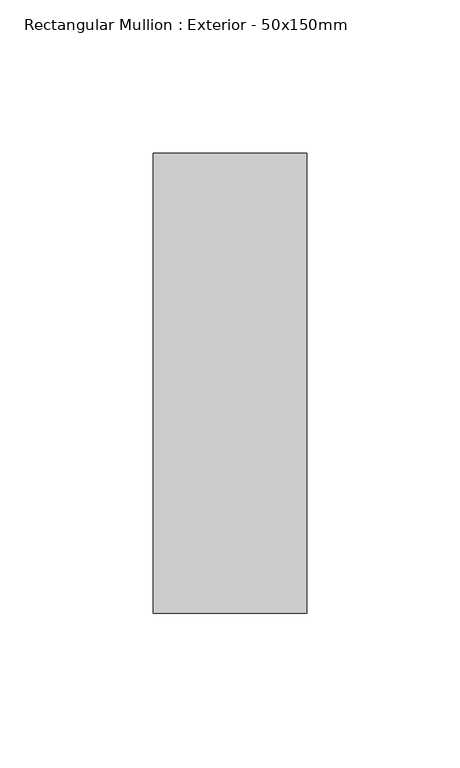
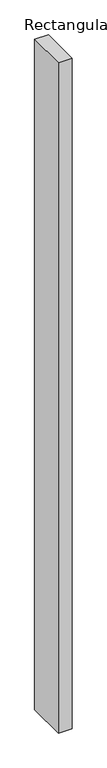
"""IFC4 building model written with IfcOpenShell, lengths in millimetres: member geometry, Rectangular Mullion : Exterior - 50x150mm."""

import ifcopenshell
import ifcopenshell.guid

model = None  # the IFC model being written
_history = None  # IfcOwnerHistory: only IFC2X3 demands one
_inside = {}  # id of a spatial element -> (the spatial element, [elements in it])
_under = {}  # id of a project, library or spatial element -> (it, [spatial elements below it])
_declared = {}  # id of a project -> (the project, [libraries it declares])
_typed = {}  # id of a type object -> (the type object, [elements of that type])
_made_of = {}  # id of a material, layer set ... -> (it, [elements and type objects made of it])


def new_model(schema):
    """Start an empty IFC model of exactly this schema.

    Asked for "IFC4X3", IfcOpenShell would pick the latest addendum, in which some entities
    have other attributes; the version numbers below select the first issue.
    IFC2X3 requires an IfcOwnerHistory on every rooted entity: one is made here for all.
    """
    global model, _history
    if schema == "IFC4X3":
        model = ifcopenshell.file(schema_version=(4, 3, 0, 0))
    else:
        model = ifcopenshell.file(schema=schema)
    _inside.clear()
    _under.clear()
    _declared.clear()
    _typed.clear()
    _made_of.clear()
    _history = None
    if model.schema == "IFC2X3":
        org = make("IfcOrganization", Name="unknown")
        user = make(
            "IfcPersonAndOrganization",
            ThePerson=make("IfcPerson", FamilyName="unknown"),
            TheOrganization=org,
        )
        app = make(
            "IfcApplication",
            ApplicationDeveloper=org,
            Version="unknown",
            ApplicationFullName="unknown",
            ApplicationIdentifier="unknown",
        )
        _history = make(
            "IfcOwnerHistory",
            OwningUser=user,
            OwningApplication=app,
            ChangeAction="ADDED",
            CreationDate=0,
        )
    return model


def make(cls, **values):
    """One entity of the class cls with the attributes given. An attribute that is None is left unset."""
    return model.create_entity(
        cls, **{name: value for name, value in values.items() if value is not None}
    )


def rooted(cls, **values):
    """An entity with a GlobalId (a new one), such as an element, a storey or a relation."""
    return make(cls, GlobalId=ifcopenshell.guid.new(), OwnerHistory=_history, **values)


def si_unit(unit_type, name, prefix=None):
    """IfcSIUnit, for example si_unit("LENGTHUNIT", "METRE", prefix="MILLI")."""
    return make("IfcSIUnit", UnitType=unit_type, Prefix=prefix, Name=name)


def assignment(units):
    """IfcUnitAssignment: the units of a project."""
    return None if units is None else make("IfcUnitAssignment", Units=units)


def point(xyz):
    """IfcCartesianPoint."""
    return None if xyz is None else make("IfcCartesianPoint", Coordinates=xyz)


def direction(xyz):
    """IfcDirection."""
    return None if xyz is None else make("IfcDirection", DirectionRatios=xyz)


def frame(location, z_axis=None, x_axis=None):
    """IfcAxis2Placement3D, a coordinate frame: its origin and axes. An axis left out is left unset."""
    return make(
        "IfcAxis2Placement3D",
        Location=point(location),
        Axis=direction(z_axis),
        RefDirection=direction(x_axis),
    )


def origin():
    """The frame at (0, 0, 0) with its axes left unset."""
    return frame((0.0, 0.0, 0.0))


def place(relative_to, where):
    """IfcLocalPlacement: puts the frame where relative to a parent placement (None: the world)."""
    return make(
        "IfcLocalPlacement", PlacementRelTo=relative_to, RelativePlacement=where
    )


def context(
    kind, dimensions, precision=None, world=None, true_north=None, identifier=None
):
    """IfcGeometricRepresentationContext, for example the 3D "Model" context."""
    return make(
        "IfcGeometricRepresentationContext",
        ContextIdentifier=identifier,
        ContextType=kind,
        CoordinateSpaceDimension=dimensions,
        Precision=precision,
        WorldCoordinateSystem=world,
        TrueNorth=true_north,
    )


def project(units=None, contexts=None):
    """IfcProject with its units and contexts."""
    return rooted(
        "IfcProject",
        Name="project",
        RepresentationContexts=contexts,
        UnitsInContext=assignment(units),
    )


def spatial(cls, under=None, at=None, **own):
    """A site, building, storey or space (cls), placed at a placement, below another one or the project."""
    s = rooted(cls, ObjectPlacement=at, **own)
    if under is not None:
        _under.setdefault(under.id(), (under, []))[1].append(s)
    return s


def polyline(points):
    """IfcPolyline through the points."""
    return make("IfcPolyline", Points=[point(p) for p in points])


def outline(outer, holes=None, kind="AREA"):
    """IfcArbitraryClosedProfileDef: a profile drawn as a closed curve; with holes, ...WithVoids."""
    if holes is None:
        return make("IfcArbitraryClosedProfileDef", ProfileType=kind, OuterCurve=outer)
    return make(
        "IfcArbitraryProfileDefWithVoids",
        ProfileType=kind,
        OuterCurve=outer,
        InnerCurves=holes,
    )


def extrude(swept, where, along, depth):
    """IfcExtrudedAreaSolid: the profile swept, set in the frame where, extruded along a direction by depth."""
    return make(
        "IfcExtrudedAreaSolid",
        SweptArea=swept,
        Position=where,
        ExtrudedDirection=direction(along),
        Depth=depth,
    )


def shape(context_of_items, identifier, shape_type, items):
    """IfcShapeRepresentation: the items that make up one representation, for example the "Body"."""
    return make(
        "IfcShapeRepresentation",
        ContextOfItems=context_of_items,
        RepresentationIdentifier=identifier,
        RepresentationType=shape_type,
        Items=items,
    )


def source(mapping_origin, context_of_items, identifier, shape_type, items):
    """IfcRepresentationMap: a shape defined once, which mapped items show again and again."""
    return make(
        "IfcRepresentationMap",
        MappingOrigin=mapping_origin,
        MappedRepresentation=shape(context_of_items, identifier, shape_type, items),
    )


def transform(
    local_origin,
    x_axis=None,
    y_axis=None,
    z_axis=None,
    scale=None,
    scale2=None,
    scale3=None,
    uniform=True,
):
    """IfcCartesianTransformationOperator3D, or its non-uniform kind. x_axis, y_axis, z_axis: its Axis1, 2, 3."""
    if uniform:
        return make(
            "IfcCartesianTransformationOperator3D",
            Axis1=direction(x_axis),
            Axis2=direction(y_axis),
            LocalOrigin=point(local_origin),
            Scale=scale,
            Axis3=direction(z_axis),
        )
    return make(
        "IfcCartesianTransformationOperator3DnonUniform",
        Axis1=direction(x_axis),
        Axis2=direction(y_axis),
        LocalOrigin=point(local_origin),
        Scale=scale,
        Axis3=direction(z_axis),
        Scale2=scale2,
        Scale3=scale3,
    )


def mapped(mapping_source, mapping_target):
    """IfcMappedItem: shows the shape of a source again, moved by a transform."""
    return make(
        "IfcMappedItem", MappingSource=mapping_source, MappingTarget=mapping_target
    )


def made_of(thing, what):
    """Note that an element or type object is made of a material, layer set ...; save() writes the relation."""
    if what is not None:
        _made_of.setdefault(what.id(), (what, []))[1].append(thing)
    return thing


def element(
    cls,
    number,
    at=None,
    inside=None,
    cuts=None,
    type_object=None,
    material=None,
    context=None,
    identifier="Body",
    shape_type=None,
    held_by="IfcProductDefinitionShape",
    body=None,
    shapes=None,
    **own,
):
    """One element of the class cls, such as IfcWall. Its Tag is "e" and its number.

    at: its placement. inside: the storey or other place that contains it. cuts: it is an
    opening in that element (IfcRelVoidsElement). A single representation is given by context,
    identifier, shape_type and body (its items); several are given by shapes. held_by: the class
    of the entity that holds the representations. save() writes the other relations.
    """
    e = rooted(cls, Tag="e%d" % number, ObjectPlacement=at, **own)
    if body is not None:
        shapes = [shape(context, identifier, shape_type, body)]
    if shapes is not None:
        e.Representation = make(held_by, Representations=shapes)
    if inside is not None:
        _inside.setdefault(inside.id(), (inside, []))[1].append(e)
    if cuts is not None:
        rooted(
            "IfcRelVoidsElement", RelatingBuildingElement=cuts, RelatedOpeningElement=e
        )
    if type_object is not None:
        _typed.setdefault(type_object.id(), (type_object, []))[1].append(e)
    return made_of(e, material)


def aggregate(whole, parts):
    """IfcRelAggregates: a whole, such as a stair, and the parts it consists of."""
    return rooted("IfcRelAggregates", RelatingObject=whole, RelatedObjects=parts)


def save(model, path):
    """Write the relations noted so far, then the file.

    IfcRelAggregates (storeys below a building ...), IfcRelContainedInSpatialStructure (elements
    in a storey), IfcRelDefinesByType, IfcRelAssociatesMaterial and IfcRelDeclares: one each for
    every whole, place, type object, material and project.
    """
    for whole, parts in _under.values():
        aggregate(whole, parts)
    for where, things in _inside.values():
        rooted(
            "IfcRelContainedInSpatialStructure",
            RelatedElements=things,
            RelatingStructure=where,
        )
    for kind, things in _typed.values():
        rooted("IfcRelDefinesByType", RelatedObjects=things, RelatingType=kind)
    for what, things in _made_of.values():
        rooted("IfcRelAssociatesMaterial", RelatedObjects=things, RelatingMaterial=what)
    for by, libraries in _declared.values():
        rooted("IfcRelDeclares", RelatingContext=by, RelatedDefinitions=libraries)
    model.write(path)


def rectangular_mullion_exterior_50x150mm_9e283e44(model_context):
    return source(origin(), model_context, "Body", "SweptSolid", [
        extrude(outline(polyline([(0.0, 0.0), (0.0, -150.0), (-50.0, -150.0), (-50.0, 0.0), (0.0, 0.0)])), frame((0.0, 0.0, -2600.0), z_axis=(0.0, 0.0, 1.0), x_axis=(1.0, 0.0, 0.0)), (0.0, 0.0, 1.0), 2600.0),
    ])


if __name__ == "__main__":
    model = new_model("IFC4")
    model_context = context("Model", 3, world=origin())
    ifc_project = project(units=[si_unit("LENGTHUNIT", "METRE", prefix="MILLI")], contexts=[model_context])
    site = spatial("IfcSite", under=ifc_project)
    building = spatial("IfcBuilding", under=site)
    placement = place(None, origin())
    rectangular_mullion_exterior_50x150mm_shape = rectangular_mullion_exterior_50x150mm_9e283e44(model_context)
    element("IfcMember", 1, ObjectType="Rectangular Mullion : Exterior - 50x150mm", at=placement, inside=building, context=model_context, shape_type="MappedRepresentation", body=[
        mapped(rectangular_mullion_exterior_50x150mm_shape, transform((0.0, 0.0, 0.0), x_axis=(1.0, 0.0, 0.0), y_axis=(0.0, 1.0, 0.0), z_axis=(0.0, 0.0, 1.0))),
    ])
    save(model, "model.ifc")

# Revit data of these elements
# Type "Rectangular Mullion : Exterior - 50x150mm"
#   built-in parameter 1007351 = -0.246063 (stored number, unit not read)
#   built-in parameter 1007304 = 0.492126 (stored number, unit not read)
#   built-in parameter 1007301 = 0.082021 (stored number, unit not read)
#   built-in parameter 1007300 = 0.082021 (stored number, unit not read)
# Element 1 (IfcMember, "Rectangular Mullion : Exterior - 50x150mm")
#   Materials on its faces: "Default Frame/Mullion (Interior/Exterior)"
# Materials
#   "Default Frame/Mullion (Interior/Exterior)": class "Generic", colour RGB 205 205 205, transparency 0, Description = "Udefineret karm/ramme materiale", Cost = 0
